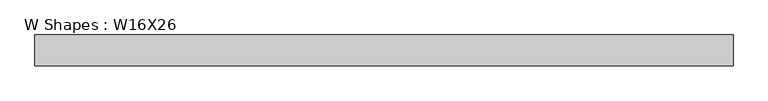
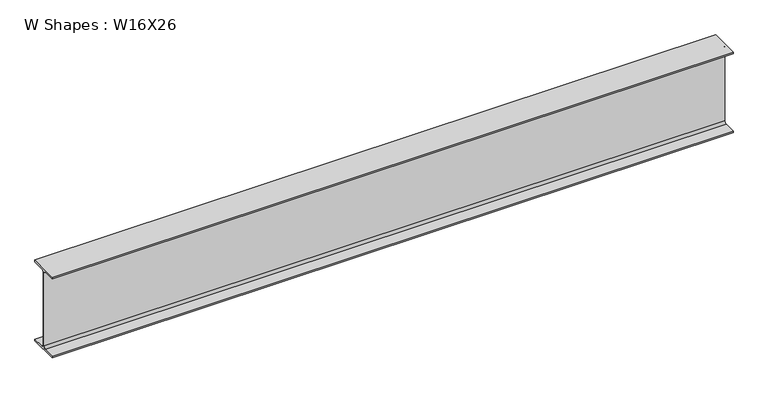
"""IFC4 building model written with IfcOpenShell, lengths in millimetres: beam geometry, W Shapes : W16X26."""

from ifc_helpers import new_model, si_unit, point, frame, frame_2d, origin, place, context, project, spatial, polyline, circle_curve, trimmed, segment, composite_curve, outline, extrude, source, transform, mapped, element, save


def w_shapes_w16x26_fcd2c860(model_context):
    return source(origin(), model_context, "Body", "SweptSolid", [
        extrude(outline(composite_curve([segment(polyline([(69.85, -190.627), (69.85, -199.39), (-69.85, -199.39), (-69.85, -190.627), (-13.3858, -190.627)]), True, "CONTINUOUS"), segment(trimmed(circle_curve(frame_2d((-13.3858, -180.4162)), 10.2108), [point((-13.3858, -190.627))], [point((-3.175, -180.4162))], True, "CARTESIAN"), True, "CONTINUOUS"), segment(polyline([(-3.175, -180.4162), (-3.175, 180.4162)]), True, "CONTINUOUS"), segment(trimmed(circle_curve(frame_2d((-13.3858, 180.4162)), 10.2108), [point((-3.175, 180.4162))], [point((-13.3858, 190.627))], True, "CARTESIAN"), True, "CONTINUOUS"), segment(polyline([(-13.3858, 190.627), (-69.85, 190.627), (-69.85, 199.39), (69.85, 199.39), (69.85, 190.627), (13.3858, 190.627)]), True, "CONTINUOUS"), segment(trimmed(circle_curve(frame_2d((13.3858, 180.4162)), 10.2108), [point((13.3858, 190.627))], [point((3.175, 180.4162))], True, "CARTESIAN"), True, "CONTINUOUS"), segment(polyline([(3.175, 180.4162), (3.175, -180.4162)]), True, "CONTINUOUS"), segment(trimmed(circle_curve(frame_2d((13.3858, -180.4162)), 10.2108), [point((3.175, -180.4162))], [point((13.3858, -190.627))], True, "CARTESIAN"), True, "CONTINUOUS"), segment(polyline([(13.3858, -190.627), (69.85, -190.627)]), True, "CONTINUOUS")], self_intersect=False)), frame((-1587.5, 0.0, 0.0), z_axis=(1.0, 0.0, 0.0), x_axis=(0.0, 1.0, 0.0)), (0.0, 0.0, 1.0), 3175.0),
    ])


if __name__ == "__main__":
    model = new_model("IFC4")
    model_context = context("Model", 3, world=origin())
    ifc_project = project(units=[si_unit("LENGTHUNIT", "METRE", prefix="MILLI")], contexts=[model_context])
    site = spatial("IfcSite", under=ifc_project)
    building = spatial("IfcBuilding", under=site)
    placement = place(None, origin())
    w_shapes_w16x26_shape = w_shapes_w16x26_fcd2c860(model_context)
    element("IfcBeam", 1, ObjectType="W Shapes : W16X26", at=placement, inside=building, context=model_context, shape_type="MappedRepresentation", body=[
        mapped(w_shapes_w16x26_shape, transform((0.0, 0.0, 0.0), x_axis=(1.0, 0.0, 0.0), y_axis=(0.0, 1.0, 0.0), z_axis=(0.0, 0.0, 1.0))),
    ])
    save(model, "model.ifc")

# Revit data of these elements
# Type "W Shapes : W16X26"
#   Section Name Key = "W16x26"
#   Assembly Code = "B10"
#   Width = 5.500"
#   Web Thickness = 0.250"
#   Web Fillet = 0.402"
#   Warping Constant = 565.00 in⁶
#   Torsional Moment of Inertia = 0.262 in⁴
#   Section Area = 7.68 in²
#   Plastic Modulus weak axis = 5.48 in³
#   Plastic Modulus strong axis = 44.20 in³
#   Perimeter = 4.35 ft²/ft
#   Nominal Weight = 26.00 lbf/ft
#   Moment of Inertia weak axis = 9.59 in⁴
#   Moment of Inertia strong axis = 301.00 in⁴
#   Height = 15.700"
#   Flange Thickness = 0.345"
#   Elastic Modulus weak axis = 3.49 in³
#   Elastic Modulus strong axis = 38.40 in³
#   Centroid Vertical = 7.850"
#   Centroid Horizontal = 2.750"
#   Bolt Spacing = 0' - 3 1/2"
#   Length [instance default] = 5' - 0"
#   Structural Material [instance default] = Steel ASTM A992
#   Principal Axes Angle = 0
# Element 1 (IfcBeam, "W Shapes : W16X26")
#   Structural Material = Steel ASTM A36
#   Materials on its faces: "Steel ASTM A36"
# Materials
#   "Steel ASTM A992": class "Metal", colour RGB 199 199 199, transparency 0, Description = "Structural steel 50ksi", Cost = 0
#   "Steel ASTM A36": class "Metal", colour RGB 199 199 199, transparency 0, Description = "Structural steel, ASTM A36 Grade B, mill finish", Cost = 0
